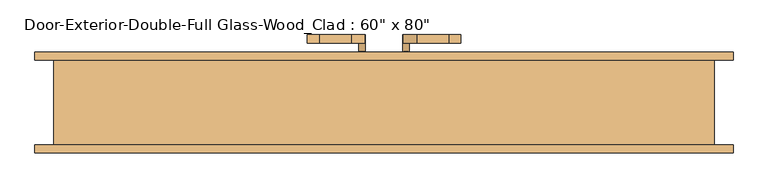
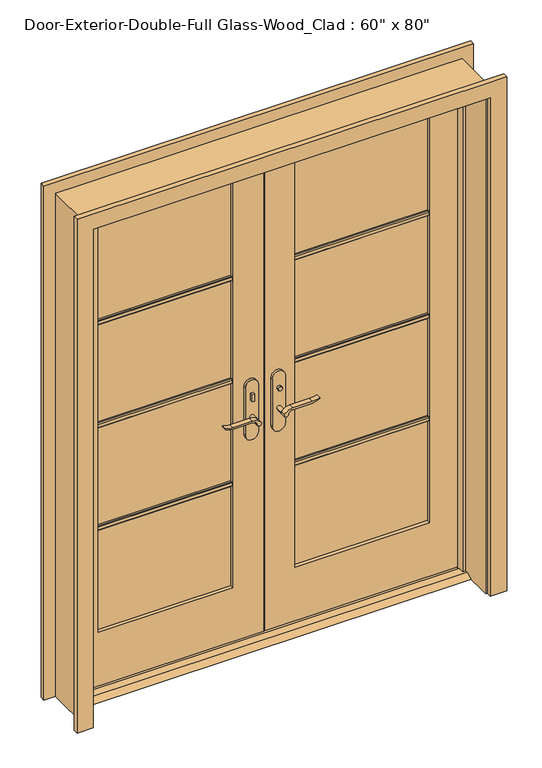
"""IFC4 building model written with IfcOpenShell, lengths in millimetres: door geometry."""

from ifc_helpers import new_model, si_unit, point, frame, frame_2d, origin, place, context, project, spatial, polyline, circle_curve, trimmed, segment, composite_curve, outline, extrude, faceted_brep, source, transform, mapped, element, save


def door_8f7b1e5f(model_context):
    return source(origin(), model_context, "Body", "SolidModel", [
        extrude(outline(polyline([(19.05, 12.7), (53.975, 12.7), (79.375, 0.0), (-6.35, 0.0), (19.05, 12.7)])), frame((-762.0, 0.0, 0.0), z_axis=(1.0, 0.0, 0.0), x_axis=(0.0, 1.0, 0.0)), (0.0, 0.0, 1.0), 1524.0),
        extrude(outline(polyline([(-47.4019111, 43.5), (-57.4019111, 43.5), (-57.4019111, 53.5), (-47.4019111, 53.5), (-47.4019111, 43.5)])), frame((0.0, 0.0, 981.9), z_axis=(0.0, 0.0, 1.0), x_axis=(1.0, 0.0, 0.0)), (0.0, 0.0, 1.0), 30.0),
        extrude(outline(composite_curve([segment(trimmed(circle_curve(frame_2d((996.9, -52.4019111)), 8.0), [point((996.9, -60.4019111))], [point((996.9, -44.4019111))], False, "CARTESIAN"), True, "CONTINUOUS"), segment(trimmed(circle_curve(frame_2d((996.9, -52.4019111)), 8.0), [point((996.9, -44.4019111))], [point((996.9, -60.4019111))], False, "CARTESIAN"), True, "CONTINUOUS")], self_intersect=False)), frame((0.0, 108.425, 0.0), z_axis=(0.0, 1.0, 0.0), x_axis=(0.0, 0.0, 1.0)), (0.0, 0.0, 1.0), 10.0),
        extrude(outline(composite_curve([segment(trimmed(circle_curve(frame_2d((897.1555521, -76.0694241)), 37.2832219), [point((919.0523287, -45.8937749))], [point((934.4, -77.7693445))], False, "CARTESIAN"), True, "CONTINUOUS"), segment(polyline([(934.4, -77.7693445), (934.4, -154.045502)]), True, "CONTINUOUS"), segment(trimmed(circle_curve(frame_2d((1017.6850638, -153.9791202)), 83.2850902), [point((934.4, -154.045502))], [point((939.4, -182.4019111))], True, "CARTESIAN"), True, "CONTINUOUS"), segment(polyline([(939.4, -182.4019111), (936.6135558, -182.4019111)]), True, "CONTINUOUS"), segment(trimmed(circle_curve(frame_2d((986.6709207, -150.4622499)), 59.3791355), [point((936.6135558, -182.4019111))], [point((927.4, -154.045502))], False, "CARTESIAN"), True, "CONTINUOUS"), segment(polyline([(927.4, -154.045502), (927.4, -77.7881013)]), True, "CONTINUOUS"), segment(trimmed(circle_curve(frame_2d((909.2738613, -77.7881013)), 18.1261387), [point((927.4, -77.7881013))], [point((914.4, -60.4019111))], True, "CARTESIAN"), True, "CONTINUOUS"), segment(trimmed(circle_curve(frame_2d((914.4, -52.4019111)), 8.0), [point((914.4, -60.4019111))], [point((919.0523287, -45.8937749))], False, "CARTESIAN"), True, "CONTINUOUS")], self_intersect=False)), frame((0.0, 3.5, 0.0), z_axis=(0.0, 1.0, 0.0), x_axis=(0.0, 0.0, 1.0)), (0.0, 0.0, 1.0), 20.0),
        extrude(outline(composite_curve([segment(trimmed(circle_curve(frame_2d((914.4, -52.4019111)), 8.0), [point((914.3999903, -60.4019111))], [point((919.0523287, -45.8937749))], False, "CARTESIAN"), True, "CONTINUOUS"), segment(trimmed(circle_curve(frame_2d((897.1555521, -76.0694241)), 37.2832219), [point((919.0523287, -45.8937749))], [point((934.4, -77.7693445))], False, "CARTESIAN"), True, "CONTINUOUS"), segment(polyline([(934.4, -77.7693445), (934.4, -154.045502)]), True, "CONTINUOUS"), segment(trimmed(circle_curve(frame_2d((1017.6850638, -153.9791202)), 83.2850902), [point((934.4, -154.045502))], [point((939.4, -182.4019111))], True, "CARTESIAN"), True, "CONTINUOUS"), segment(polyline([(939.4, -182.4019111), (936.6135558, -182.4019111)]), True, "CONTINUOUS"), segment(trimmed(circle_curve(frame_2d((986.6709207, -150.4622499)), 59.3791355), [point((936.6135558, -182.4019111))], [point((927.4, -154.045502))], False, "CARTESIAN"), True, "CONTINUOUS"), segment(polyline([(927.4, -154.045502), (927.4, -77.788099)]), True, "CONTINUOUS"), segment(trimmed(circle_curve(frame_2d((909.2738682, -77.788099)), 18.1261318), [point((927.4, -77.788099))], [point((914.3999903, -60.4019111))], True, "CARTESIAN"), True, "CONTINUOUS")], self_intersect=False)), frame((0.0, 138.425, 0.0), z_axis=(0.0, 1.0, 0.0), x_axis=(0.0, 0.0, 1.0)), (0.0, 0.0, 1.0), 20.0),
        extrude(outline(composite_curve([segment(trimmed(circle_curve(frame_2d((914.4, -52.4019111)), 8.0), [point((914.4, -60.4019111))], [point((914.4, -44.4019111))], False, "CARTESIAN"), True, "CONTINUOUS"), segment(trimmed(circle_curve(frame_2d((914.4, -52.4019111)), 8.0), [point((914.4, -44.4019111))], [point((914.4, -60.4019111))], False, "CARTESIAN"), True, "CONTINUOUS")], self_intersect=False)), frame((0.0, 23.5, 0.0), z_axis=(0.0, 1.0, 0.0), x_axis=(0.0, 0.0, 1.0)), (0.0, 0.0, 1.0), 30.0),
        extrude(outline(composite_curve([segment(trimmed(circle_curve(frame_2d((914.4, -52.4019111)), 8.0), [point((914.4, -60.4019111))], [point((914.4, -44.4019111))], False, "CARTESIAN"), True, "CONTINUOUS"), segment(trimmed(circle_curve(frame_2d((914.4, -52.4019111)), 8.0), [point((914.4, -44.4019111))], [point((914.4, -60.4019111))], False, "CARTESIAN"), True, "CONTINUOUS")], self_intersect=False)), frame((0.0, 108.425, 0.0), z_axis=(0.0, 1.0, 0.0), x_axis=(0.0, 0.0, 1.0)), (0.0, 0.0, 1.0), 30.0),
        extrude(outline(composite_curve([segment(polyline([(844.4, -27.4019111), (1039.4, -27.4019111)]), True, "CONTINUOUS"), segment(trimmed(circle_curve(frame_2d((1039.4, -52.4019111)), 25.0), [point((1039.4, -27.4019111))], [point((1039.4, -77.4019111))], False, "CARTESIAN"), True, "CONTINUOUS"), segment(polyline([(1039.4, -77.4019111), (844.4, -77.4019111)]), True, "CONTINUOUS"), segment(trimmed(circle_curve(frame_2d((844.4, -52.4019111)), 25.0), [point((844.4, -77.4019111))], [point((844.4, -27.4019111))], False, "CARTESIAN"), True, "CONTINUOUS")], self_intersect=False)), frame((0.0, 53.5, 0.0), z_axis=(0.0, 1.0, 0.0), x_axis=(0.0, 0.0, 1.0)), (0.0, 0.0, 1.0), 10.0),
        extrude(outline(composite_curve([segment(polyline([(844.4, -27.4019111), (1039.4, -27.4019111)]), True, "CONTINUOUS"), segment(trimmed(circle_curve(frame_2d((1039.4, -52.4019111)), 25.0), [point((1039.4, -27.4019111))], [point((1039.4, -77.4019111))], False, "CARTESIAN"), True, "CONTINUOUS"), segment(polyline([(1039.4, -77.4019111), (844.4, -77.4019111)]), True, "CONTINUOUS"), segment(trimmed(circle_curve(frame_2d((844.4, -52.4019111)), 25.0), [point((844.4, -77.4019111))], [point((844.4, -27.4019111))], False, "CARTESIAN"), True, "CONTINUOUS")], self_intersect=False)), frame((0.0, 98.425, 0.0), z_axis=(0.0, 1.0, 0.0), x_axis=(0.0, 0.0, 1.0)), (0.0, 0.0, 1.0), 10.0),
        extrude(outline(polyline([(47.3875, 118.425), (57.3875, 118.425), (57.3875, 108.425), (47.3875, 108.425), (47.3875, 118.425)])), frame((0.0, 0.0, 981.9), z_axis=(0.0, 0.0, 1.0), x_axis=(1.0, 0.0, 0.0)), (0.0, 0.0, 1.0), 30.0),
        extrude(outline(composite_curve([segment(trimmed(circle_curve(frame_2d((996.9, 52.3875)), 8.0), [point((996.9, 60.3875))], [point((996.9, 44.3875))], False, "CARTESIAN"), True, "CONTINUOUS"), segment(trimmed(circle_curve(frame_2d((996.9, 52.3875)), 8.0), [point((996.9, 44.3875))], [point((996.9, 60.3875))], False, "CARTESIAN"), True, "CONTINUOUS")], self_intersect=False)), frame((0.0, 43.5, 0.0), z_axis=(0.0, 1.0, 0.0), x_axis=(0.0, 0.0, 1.0)), (0.0, 0.0, 1.0), 10.0),
        extrude(outline(composite_curve([segment(trimmed(circle_curve(frame_2d((914.4, 52.3875)), 8.0), [point((919.0523287, 45.8793637))], [point((914.4, 60.3875))], False, "CARTESIAN"), True, "CONTINUOUS"), segment(trimmed(circle_curve(frame_2d((909.2738613, 77.7736901)), 18.1261387), [point((914.4, 60.3875))], [point((927.4, 77.7736901))], True, "CARTESIAN"), True, "CONTINUOUS"), segment(polyline([(927.4, 77.7736901), (927.4, 154.0310909)]), True, "CONTINUOUS"), segment(trimmed(circle_curve(frame_2d((986.6709207, 150.4478388)), 59.3791355), [point((927.4, 154.0310909))], [point((936.6135558, 182.3875))], False, "CARTESIAN"), True, "CONTINUOUS"), segment(polyline([(936.6135558, 182.3875), (939.4, 182.3875)]), True, "CONTINUOUS"), segment(trimmed(circle_curve(frame_2d((1017.6850638, 153.9647091)), 83.2850902), [point((939.4, 182.3875))], [point((934.4, 154.0310909))], True, "CARTESIAN"), True, "CONTINUOUS"), segment(polyline([(934.4, 154.0310909), (934.4, 77.7549333)]), True, "CONTINUOUS"), segment(trimmed(circle_curve(frame_2d((897.1555521, 76.0550129)), 37.2832219), [point((934.4, 77.7549333))], [point((919.0523287, 45.8793637))], False, "CARTESIAN"), True, "CONTINUOUS")], self_intersect=False)), frame((0.0, 138.425, 0.0), z_axis=(0.0, 1.0, 0.0), x_axis=(0.0, 0.0, 1.0)), (0.0, 0.0, 1.0), 20.0),
        extrude(outline(composite_curve([segment(trimmed(circle_curve(frame_2d((909.2738682, 77.7736878)), 18.1261318), [point((914.3999903, 60.3875))], [point((927.4, 77.7736878))], True, "CARTESIAN"), True, "CONTINUOUS"), segment(polyline([(927.4, 77.7736878), (927.4, 154.0310909)]), True, "CONTINUOUS"), segment(trimmed(circle_curve(frame_2d((986.6709207, 150.4478388)), 59.3791355), [point((927.4, 154.0310909))], [point((936.6135558, 182.3875))], False, "CARTESIAN"), True, "CONTINUOUS"), segment(polyline([(936.6135558, 182.3875), (939.4, 182.3875)]), True, "CONTINUOUS"), segment(trimmed(circle_curve(frame_2d((1017.6850638, 153.9647091)), 83.2850902), [point((939.4, 182.3875))], [point((934.4, 154.0310909))], True, "CARTESIAN"), True, "CONTINUOUS"), segment(polyline([(934.4, 154.0310909), (934.4, 77.7549333)]), True, "CONTINUOUS"), segment(trimmed(circle_curve(frame_2d((897.1555521, 76.0550129)), 37.2832219), [point((934.4, 77.7549333))], [point((919.0523287, 45.8793637))], False, "CARTESIAN"), True, "CONTINUOUS"), segment(trimmed(circle_curve(frame_2d((914.4, 52.3875)), 8.0), [point((919.0523287, 45.8793637))], [point((914.3999903, 60.3875))], False, "CARTESIAN"), True, "CONTINUOUS")], self_intersect=False)), frame((0.0, 3.5, 0.0), z_axis=(0.0, 1.0, 0.0), x_axis=(0.0, 0.0, 1.0)), (0.0, 0.0, 1.0), 20.0),
        extrude(outline(composite_curve([segment(trimmed(circle_curve(frame_2d((914.4, 52.3875)), 8.0), [point((914.4, 60.3875))], [point((914.4, 44.3875))], False, "CARTESIAN"), True, "CONTINUOUS"), segment(trimmed(circle_curve(frame_2d((914.4, 52.3875)), 8.0), [point((914.4, 44.3875))], [point((914.4, 60.3875))], False, "CARTESIAN"), True, "CONTINUOUS")], self_intersect=False)), frame((0.0, 108.425, 0.0), z_axis=(0.0, 1.0, 0.0), x_axis=(0.0, 0.0, 1.0)), (0.0, 0.0, 1.0), 30.0),
        extrude(outline(composite_curve([segment(trimmed(circle_curve(frame_2d((914.4, 52.3875)), 8.0), [point((914.4, 60.3875))], [point((914.4, 44.3875))], False, "CARTESIAN"), True, "CONTINUOUS"), segment(trimmed(circle_curve(frame_2d((914.4, 52.3875)), 8.0), [point((914.4, 44.3875))], [point((914.4, 60.3875))], False, "CARTESIAN"), True, "CONTINUOUS")], self_intersect=False)), frame((0.0, 23.5, 0.0), z_axis=(0.0, 1.0, 0.0), x_axis=(0.0, 0.0, 1.0)), (0.0, 0.0, 1.0), 30.0),
        extrude(outline(composite_curve([segment(trimmed(circle_curve(frame_2d((844.4, 52.3875)), 25.0), [point((844.4, 27.3875))], [point((844.4, 77.3875))], False, "CARTESIAN"), True, "CONTINUOUS"), segment(polyline([(844.4, 77.3875), (1039.4, 77.3875)]), True, "CONTINUOUS"), segment(trimmed(circle_curve(frame_2d((1039.4, 52.3875)), 25.0), [point((1039.4, 77.3875))], [point((1039.4, 27.3875))], False, "CARTESIAN"), True, "CONTINUOUS"), segment(polyline([(1039.4, 27.3875), (844.4, 27.3875)]), True, "CONTINUOUS")], self_intersect=False)), frame((0.0, 98.425, 0.0), z_axis=(0.0, 1.0, 0.0), x_axis=(0.0, 0.0, 1.0)), (0.0, 0.0, 1.0), 10.0),
        extrude(outline(composite_curve([segment(trimmed(circle_curve(frame_2d((844.4, 52.3875)), 25.0), [point((844.4, 27.3875))], [point((844.4, 77.3875))], False, "CARTESIAN"), True, "CONTINUOUS"), segment(polyline([(844.4, 77.3875), (1039.4, 77.3875)]), True, "CONTINUOUS"), segment(trimmed(circle_curve(frame_2d((1039.4, 52.3875)), 25.0), [point((1039.4, 77.3875))], [point((1039.4, 27.3875))], False, "CARTESIAN"), True, "CONTINUOUS"), segment(polyline([(1039.4, 27.3875), (844.4, 27.3875)]), True, "CONTINUOUS")], self_intersect=False)), frame((0.0, 53.5, 0.0), z_axis=(0.0, 1.0, 0.0), x_axis=(0.0, 0.0, 1.0)), (0.0, 0.0, 1.0), 10.0),
        extrude(outline(polyline([(77.47, 1502.171875), (77.47, 1483.121875), (71.12, 1483.121875), (67.945, 1486.296875), (67.945, 1498.996875), (71.12, 1502.171875), (77.47, 1502.171875)])), frame((120.65, 0.0, 0.0), z_axis=(1.0, 0.0, 0.0), x_axis=(0.0, 1.0, 0.0)), (0.0, 0.0, 1.0), 520.7),
        extrude(outline(polyline([(77.47, 1081.88125), (77.47, 1062.83125), (71.12, 1062.83125), (67.945, 1066.00625), (67.945, 1078.70625), (71.12, 1081.88125), (77.47, 1081.88125)])), frame((120.65, 0.0, 0.0), z_axis=(1.0, 0.0, 0.0), x_axis=(0.0, 1.0, 0.0)), (0.0, 0.0, 1.0), 520.7),
        extrude(outline(polyline([(77.47, 661.590625), (77.47, 642.540625), (71.12, 642.540625), (67.945, 645.715625), (67.945, 658.415625), (71.12, 661.590625), (77.47, 661.590625)])), frame((120.65, 0.0, 0.0), z_axis=(1.0, 0.0, 0.0), x_axis=(0.0, 1.0, 0.0)), (0.0, 0.0, 1.0), 520.7),
        extrude(outline(polyline([(84.455, 1502.171875), (90.805, 1502.171875), (93.98, 1498.996875), (93.98, 1486.296875), (90.805, 1483.121875), (84.455, 1483.121875), (84.455, 1502.171875)])), frame((-641.35, 0.0, 0.0), z_axis=(1.0, 0.0, 0.0), x_axis=(0.0, 1.0, 0.0)), (0.0, 0.0, 1.0), 520.7),
        extrude(outline(polyline([(84.455, 1081.88125), (90.805, 1081.88125), (93.98, 1078.70625), (93.98, 1066.00625), (90.805, 1062.83125), (84.455, 1062.83125), (84.455, 1081.88125)])), frame((-641.35, 0.0, 0.0), z_axis=(1.0, 0.0, 0.0), x_axis=(0.0, 1.0, 0.0)), (0.0, 0.0, 1.0), 520.7),
        extrude(outline(polyline([(84.455, 661.590625), (90.805, 661.590625), (93.98, 658.415625), (93.98, 645.715625), (90.805, 642.540625), (84.455, 642.540625), (84.455, 661.590625)])), frame((-641.35, 0.0, 0.0), z_axis=(1.0, 0.0, 0.0), x_axis=(0.0, 1.0, 0.0)), (0.0, 0.0, 1.0), 520.7),
        extrude(outline(polyline([(84.455, 1502.171875), (90.805, 1502.171875), (93.98, 1498.996875), (93.98, 1486.296875), (90.805, 1483.121875), (84.455, 1483.121875), (84.455, 1502.171875)])), frame((120.65, 0.0, 0.0), z_axis=(1.0, 0.0, 0.0), x_axis=(0.0, 1.0, 0.0)), (0.0, 0.0, 1.0), 520.7),
        extrude(outline(polyline([(84.455, 1081.88125), (90.805, 1081.88125), (93.98, 1078.70625), (93.98, 1066.00625), (90.805, 1062.83125), (84.455, 1062.83125), (84.455, 1081.88125)])), frame((120.65, 0.0, 0.0), z_axis=(1.0, 0.0, 0.0), x_axis=(0.0, 1.0, 0.0)), (0.0, 0.0, 1.0), 520.7),
        extrude(outline(polyline([(84.455, 661.590625), (90.805, 661.590625), (93.98, 658.415625), (93.98, 645.715625), (90.805, 642.540625), (84.455, 642.540625), (84.455, 661.590625)])), frame((120.65, 0.0, 0.0), z_axis=(1.0, 0.0, 0.0), x_axis=(0.0, 1.0, 0.0)), (0.0, 0.0, 1.0), 520.7),
        extrude(outline(polyline([(77.47, 1502.171875), (77.47, 1483.121875), (71.12, 1483.121875), (67.945, 1486.296875), (67.945, 1498.996875), (71.12, 1502.171875), (77.47, 1502.171875)])), frame((-641.35, 0.0, 0.0), z_axis=(1.0, 0.0, 0.0), x_axis=(0.0, 1.0, 0.0)), (0.0, 0.0, 1.0), 520.7),
        extrude(outline(polyline([(77.47, 1081.88125), (77.47, 1062.83125), (71.12, 1062.83125), (67.945, 1066.00625), (67.945, 1078.70625), (71.12, 1081.88125), (77.47, 1081.88125)])), frame((-641.35, 0.0, 0.0), z_axis=(1.0, 0.0, 0.0), x_axis=(0.0, 1.0, 0.0)), (0.0, 0.0, 1.0), 520.7),
        extrude(outline(polyline([(77.47, 661.590625), (77.47, 642.540625), (71.12, 642.540625), (67.945, 645.715625), (67.945, 658.415625), (71.12, 661.590625), (77.47, 661.590625)])), frame((-641.35, 0.0, 0.0), z_axis=(1.0, 0.0, 0.0), x_axis=(0.0, 1.0, 0.0)), (0.0, 0.0, 1.0), 520.7),
        extrude(outline(polyline([(0.0, 768.35), (0.0, 831.85), (2101.85, 831.85), (2101.85, -831.85), (0.0, -831.85), (0.0, -768.35), (2038.35, -768.35), (2038.35, 768.35), (0.0, 768.35)])), frame((0.0, 98.425, 0.0), z_axis=(0.0, 1.0, 0.0), x_axis=(0.0, 0.0, 1.0)), (0.0, 0.0, 1.0), 19.05),
        extrude(outline(polyline([(0.0, 768.35), (0.0, 831.85), (2101.85, 831.85), (2101.85, -831.85), (0.0, -831.85), (0.0, -768.35), (2038.35, -768.35), (2038.35, 768.35), (0.0, 768.35)])), frame((0.0, -123.825, 0.0), z_axis=(0.0, 1.0, 0.0), x_axis=(0.0, 0.0, 1.0)), (0.0, 0.0, 1.0), 19.05),
        extrude(outline(polyline([(12.7, 762.0), (2032.0, 762.0), (2032.0, 1.5875), (12.7, 1.5875), (12.7, 762.0)]), holes=[polyline([(1912.9375, 120.65), (1912.9375, 641.35), (231.775, 641.35), (231.775, 120.65), (1912.9375, 120.65)])]), frame((0.0, 63.5, 0.0), z_axis=(0.0, 1.0, 0.0), x_axis=(0.0, 0.0, 1.0)), (0.0, 0.0, 1.0), 34.925),
        extrude(outline(polyline([(2032.0, -762.0), (12.7, -762.0), (12.7, -1.6019111), (2032.0, -1.6019111), (2032.0, -762.0)]), holes=[polyline([(231.775, -641.35), (1912.9375, -641.35), (1912.9375, -120.65), (231.775, -120.65), (231.775, -641.35)])]), frame((0.0, 63.5, 0.0), z_axis=(0.0, 1.0, 0.0), x_axis=(0.0, 0.0, 1.0)), (0.0, 0.0, 1.0), 34.925),
        faceted_brep([(787.4, 98.425, 0.0), (787.4, -104.775, 0.0), (762.0, -104.775, 0.0), (762.0, 28.575, 0.0), (749.3, 28.575, 0.0), (749.3, 63.5, 0.0), (762.0, 63.5, 0.0), (762.0, 98.425, 0.0), (787.4, 98.425, 2057.4), (787.4, -104.775, 2057.4), (-787.4, -104.775, 2057.4), (-787.4, -104.775, 0.0), (-762.0, -104.775, 0.0), (-762.0, -104.775, 2032.0), (762.0, -104.775, 2032.0), (762.0, 28.575, 2032.0), (-762.0, 28.575, 2032.0), (-762.0, 28.575, 0.0), (-749.3, 28.575, 0.0), (-749.3, 28.575, 2019.3), (749.3, 28.575, 2019.3), (749.3, 63.5, 2019.3), (1.5875, 63.5, 2019.3), (-1.6019111, 63.5, 2019.3), (-749.3, 63.5, 2019.3), (-749.3, 63.5, 0.0), (-762.0, 63.5, 0.0), (-762.0, 63.5, 2032.0), (-1.6019111, 63.5, 2032.0), (1.5875, 63.5, 2032.0), (762.0, 63.5, 2032.0), (762.0, 98.425, 2032.0), (1.5875, 98.425, 2032.0), (-1.6019111, 98.425, 2032.0), (-762.0, 98.425, 2032.0), (-762.0, 98.425, 0.0), (-787.4, 98.425, 0.0), (-787.4, 98.425, 2057.4)], [[[0, 1, 2, 3, 4, 5, 6, 7]], [[1, 0, 8, 9]], [[2, 1, 9, 10, 11, 12, 13, 14]], [[3, 2, 14, 15]], [[4, 3, 15, 16, 17, 18, 19, 20]], [[5, 4, 20, 21]], [[6, 5, 21, 22, 23, 24, 25, 26, 27, 28, 29, 30]], [[7, 6, 30, 31]], [[0, 7, 31, 32, 33, 34, 35, 36, 37, 8]], [[9, 8, 37, 10]], [[14, 13, 16, 15]], [[20, 19, 24, 23, 22, 21]], [[31, 30, 29, 28, 27, 34, 33, 32]], [[12, 11, 36, 35, 26, 25, 18, 17]], [[11, 10, 37, 36]], [[13, 12, 17, 16]], [[19, 18, 25, 24]], [[27, 26, 35, 34]]]),
        extrude(outline(polyline([(641.35, 77.47), (120.65, 77.47), (120.65, 84.455), (641.35, 84.455), (641.35, 77.47)])), frame((0.0, 0.0, 231.775), z_axis=(0.0, 0.0, 1.0), x_axis=(1.0, 0.0, 0.0)), (0.0, 0.0, 1.0), 1681.1625),
        extrude(outline(polyline([(-120.65, 77.47), (-641.35, 77.47), (-641.35, 84.455), (-120.65, 84.455), (-120.65, 77.47)])), frame((0.0, 0.0, 231.775), z_axis=(0.0, 0.0, 1.0), x_axis=(1.0, 0.0, 0.0)), (0.0, 0.0, 1.0), 1681.1625),
    ])


if __name__ == "__main__":
    model = new_model("IFC4")
    model_context = context("Model", 3, world=origin())
    ifc_project = project(units=[si_unit("LENGTHUNIT", "METRE", prefix="MILLI")], contexts=[model_context])
    site = spatial("IfcSite", under=ifc_project)
    building = spatial("IfcBuilding", under=site)
    placement = place(None, origin())
    door_shape = door_8f7b1e5f(model_context)
    element("IfcDoor", 1, ObjectType="Door-Exterior-Double-Full Glass-Wood_Clad : 60\" x 80\"", at=placement, inside=building, context=model_context, shape_type="MappedRepresentation", body=[
        mapped(door_shape, transform((0.0, 0.0, 0.0), x_axis=(1.0, 0.0, 0.0), y_axis=(0.0, 1.0, 0.0), z_axis=(0.0, 0.0, 1.0))),
    ])
    save(model, "model.ifc")

# Revit data of these elements
# Type "Door-Exterior-Double-Full Glass-Wood_Clad : 60\" x 80\""
#   Type Mark = "8"
#   Assembly Code = "B2030100"
#   Analytic Construction = "French door, wood frame with double glass"
#   Top Rail = 0' - 4 11/16"
#   Threshold Offset [instance default] = 0' - 0 1/2"
#   Thickness = 0' - 1 3/8"
#   Thermal Resistance (R) = 1.9158 (h·ft²·°F)/BTU
#   Swing Angle [instance default] = 90.00°
#   Stiles = 0' - 4 3/4"
#   Rough Width = 5' - 2"
#   Rough Height = 6' - 9"
#   Panel Width = 2' - 6"
#   Door Offset [instance default] = 0' - 0"
#   Height = 6' - 8"
#   Width = 5' - 0"
#   Heat Transfer Coefficient (U) = 0.5220 BTU/(h·ft²·°F)
#   Bottom Rail = 0' - 9 1/8"
#   Exterior Trim [instance default] = yes
#   Threshold [instance default] = yes
#   Show Grill [instance default] = yes
#   Function = 1
#   Trim Material = Cherry
#   Threshold Material = Cherry
#   Panel Material = Cherry
#   Glazing = Glass
#   Frame Material = Cherry
#   Door Handle Material = Aluminum
#   Visual Light Transmittance = 0
#   Solar Heat Gain Coefficient = 0
#   Wall Closure = (empty or 0)
#   Construction Type = (empty or 0)
# Element 1 (IfcDoor, "Door-Exterior-Double-Full Glass-Wood_Clad : 60\" x 80\"")
#   Materials on its faces: "Cherry", "Aluminum", "Glass"
# Materials
#   "Cherry": class "Wood", colour RGB 226 177 128, transparency 0, Description = "Prunus Serotina", Cost = 0
#   "Glass": class "Glass", colour RGB 0 128 192, transparency 0.75, Description = "Soda Lime Glass", Cost = 0
#   "Aluminum": class "Metal", colour RGB 247 247 247, transparency 0, Description = "Aluminum 6061", Cost = 0
